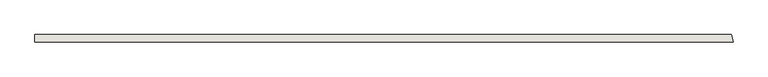
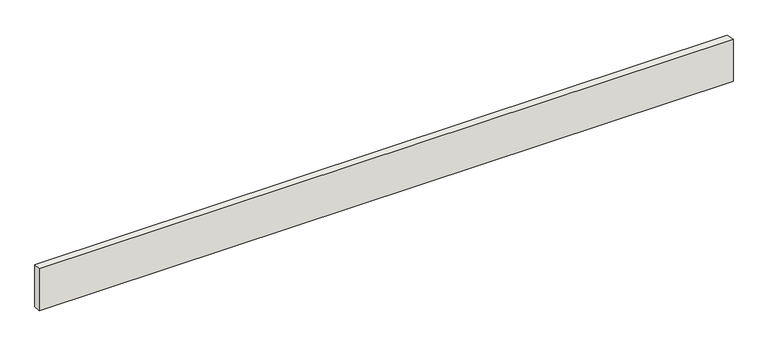
"""IFC4 building model written with IfcOpenShell, lengths in millimetres: wall geometry, Holzwand."""

from ifc_helpers import new_model, si_unit, origin, origin_with_axes, place, context, project, spatial, polyline, outline, extrude, source, transform, mapped, element, save


def wall_cfff9ef7(model_context):
    return source(origin(), model_context, "Body", "SweptSolid", [
        extrude(outline(polyline([(18752.8972975, 0.0), (0.0, 0.0), (0.1365557, 200.0), (18704.78903, 200.0), (18752.8972975, 0.0)])), origin_with_axes(), (0.0, 0.0, 1.0), 1200.0),
    ])


if __name__ == "__main__":
    model = new_model("IFC4")
    model_context = context("Model", 3, world=origin())
    ifc_project = project(units=[si_unit("LENGTHUNIT", "METRE", prefix="MILLI")], contexts=[model_context])
    site = spatial("IfcSite", under=ifc_project)
    building = spatial("IfcBuilding", under=site)
    placement = place(None, origin())
    wall_shape = wall_cfff9ef7(model_context)
    element("IfcWall", 1, ObjectType="Holzwand", at=placement, inside=building, context=model_context, shape_type="MappedRepresentation", body=[
        mapped(wall_shape, transform((0.0, 0.0, 0.0), x_axis=(1.0, 0.0, 0.0), y_axis=(0.0, 1.0, 0.0), z_axis=(0.0, 0.0, 1.0))),
    ])
    save(model, "model.ifc")

# Revit data of these elements
# Element 1 (IfcWall, "Holzwand")
#   Materials on its faces: "NC-GK-Platte-grau"
# Materials
#   "NC-GK-Platte-grau": class "Unassigned", colour RGB 199 199 199, transparency 0
